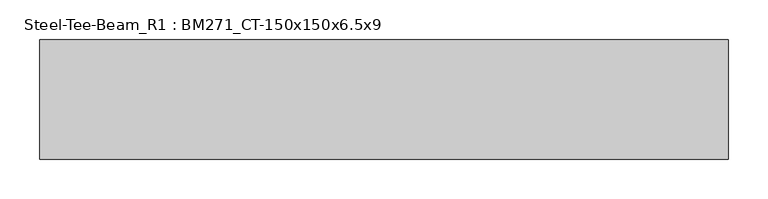
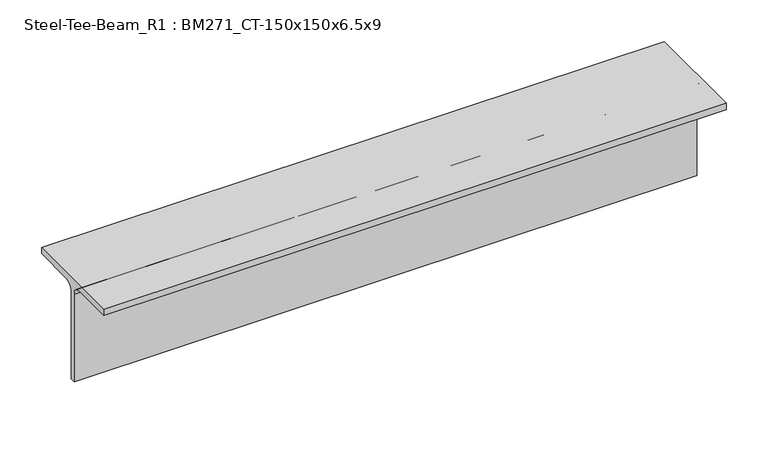
"""IFC4 building model written with IfcOpenShell, lengths in millimetres: member geometry, Steel-Tee-Beam_R1 : BM271_CT-150x150x6.5x9."""

from ifc_helpers import new_model, si_unit, point, frame, frame_2d, origin, place, context, project, spatial, polyline, circle_curve, trimmed, segment, composite_curve, outline, extrude, source, transform, mapped, element, save


def steel_tee_beam_r1_bm271_ct_150x150x6_5x9_b170fee5(model_context):
    return source(origin(), model_context, "Body", "SweptSolid", [
        extrude(outline(composite_curve([segment(polyline([(75.0, 75.0), (75.0, 66.0), (16.25, 66.0)]), True, "CONTINUOUS"), segment(trimmed(circle_curve(frame_2d((16.25, 53.0)), 13.0), [point((16.25, 66.0))], [point((3.25, 53.0))], True, "CARTESIAN"), True, "CONTINUOUS"), segment(polyline([(3.25, 53.0), (3.25, -75.0), (-3.25, -75.0), (-3.25, 53.0)]), True, "CONTINUOUS"), segment(trimmed(circle_curve(frame_2d((-16.25, 53.0)), 13.0), [point((-3.25, 53.0))], [point((-16.25, 66.0))], True, "CARTESIAN"), True, "CONTINUOUS"), segment(polyline([(-16.25, 66.0), (-75.0, 66.0), (-75.0, 75.0), (75.0, 75.0)]), True, "CONTINUOUS")], self_intersect=False)), frame((-500.0, 0.0, 0.0), z_axis=(1.0, 0.0, 0.0), x_axis=(0.0, 1.0, 0.0)), (0.0, 0.0, 1.0), 865.9474508),
    ])


if __name__ == "__main__":
    model = new_model("IFC4")
    model_context = context("Model", 3, world=origin())
    ifc_project = project(units=[si_unit("LENGTHUNIT", "METRE", prefix="MILLI")], contexts=[model_context])
    site = spatial("IfcSite", under=ifc_project)
    building = spatial("IfcBuilding", under=site)
    placement = place(None, origin())
    steel_tee_beam_r1_bm271_ct_150x150x6_5x9_shape = steel_tee_beam_r1_bm271_ct_150x150x6_5x9_b170fee5(model_context)
    element("IfcMember", 1, ObjectType="Steel-Tee-Beam_R1 : BM271_CT-150x150x6.5x9", at=placement, inside=building, context=model_context, shape_type="MappedRepresentation", body=[
        mapped(steel_tee_beam_r1_bm271_ct_150x150x6_5x9_shape, transform((0.0, 0.0, 0.0), x_axis=(1.0, 0.0, 0.0), y_axis=(0.0, 1.0, 0.0), z_axis=(0.0, 0.0, 1.0))),
    ])
    save(model, "model.ifc")

# Revit data of these elements
# Type "Steel-Tee-Beam_R1 : BM271_CT-150x150x6.5x9"
#   Keynote = "CT-150x150x6.5x9"
#   Surface Area = 0.588841 m²/m
#   Section Area = 23.3904 cm²
#   Mass per Unit Length = 18.3614 kg/m
#   Length [instance default] = 1.5240 m
#   bf = 0.1500 m
#   d = 0.1500 m
#   k = 0.0220 m
#   r = 0.0130 m
#   tf = 0.0090 m
#   tw = 0.0065 m
#   hec_material4 [instance default] = none
#   hec_material3 [instance default] = none
#   hec_material2 [instance default] = none
#   hec_material1 [instance default] = none
#   Structural Material [instance default] = Steel, 45-345
#   Assembly Code = ""
# Element 1 (IfcMember, "Steel-Tee-Beam_R1 : BM271_CT-150x150x6.5x9")
#   Structural Material = none
# Materials
#   "Steel, 45-345": class "Metal", colour RGB 189 187 185, transparency 0, Description = "Steel 345 MPa", Cost = 0
